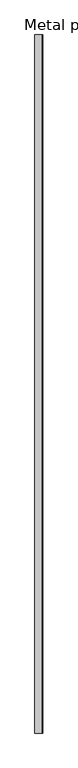
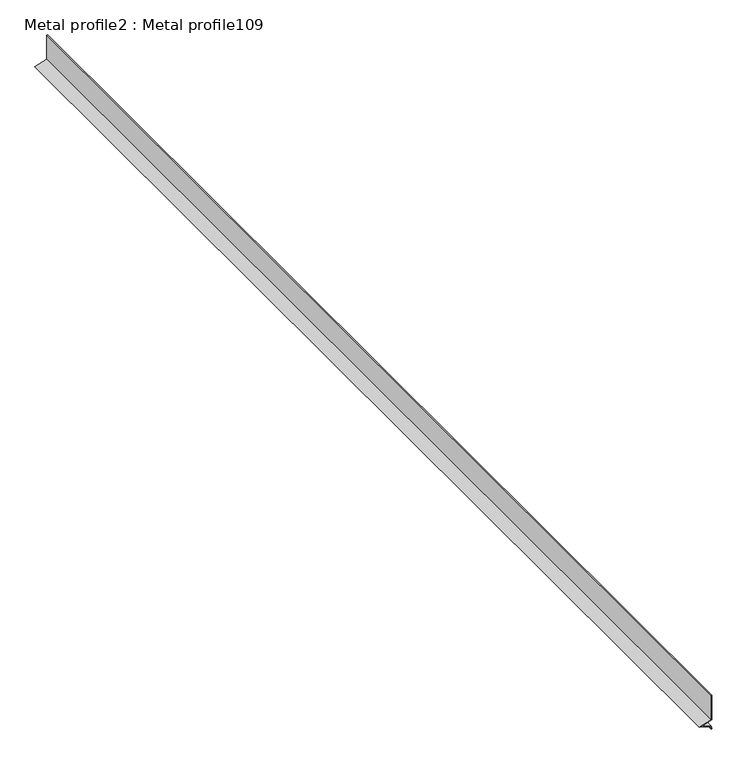
"""IFC4 building model written with IfcOpenShell, lengths in millimetres: proxy geometry, Metal profile2 : Metal profile109."""

from ifc_helpers import new_model, si_unit, frame, origin, place, context, project, spatial, polyline, outline, extrude, source, transform, mapped, element, save


def metal_profile2_metal_profile109_c648c6db(model_context):
    return source(origin(), model_context, "Body", "SweptSolid", [
        extrude(outline(polyline([(36749.8837679, 10041.7861998), (36754.9985183, 10040.8230047), (36760.4986763, 10023.7114021), (36766.3084327, 10041.7861998), (36811.2986763, 10041.7861998), (36811.2986763, 10040.5161998), (36767.234212, 10040.5161998), (36760.4986763, 10019.5611998), (36754.0207281, 10039.7148163), (36749.6487364, 10040.5381373), (36749.8837679, 10041.7861998)])), frame((0.0, 2217.3610563, 0.0), z_axis=(0.0, 1.0, 0.0), x_axis=(0.0, 0.0, 1.0)), (0.0, 0.0, 1.0), 2000.0),
    ])


if __name__ == "__main__":
    model = new_model("IFC4")
    model_context = context("Model", 3, world=origin())
    ifc_project = project(units=[si_unit("LENGTHUNIT", "METRE", prefix="MILLI")], contexts=[model_context])
    site = spatial("IfcSite", under=ifc_project)
    building = spatial("IfcBuilding", under=site)
    placement = place(None, origin())
    metal_profile2_metal_profile109_shape = metal_profile2_metal_profile109_c648c6db(model_context)
    element("IfcBuildingElementProxy", 1, Name="Metal profile2 : Metal profile109", ObjectType="Metal profile2 : Metal profile109", at=placement, inside=building, context=model_context, shape_type="MappedRepresentation", body=[
        mapped(metal_profile2_metal_profile109_shape, transform((0.0, 0.0, 0.0), x_axis=(1.0, 0.0, 0.0), y_axis=(0.0, 1.0, 0.0), z_axis=(0.0, 0.0, 1.0))),
    ])
    save(model, "model.ifc")

# Revit data of these elements
# Type "Metal profile2 : Metal profile109"
#   NameOverride = "Metal profile109"
# Element 1 (IfcBuildingElementProxy, "Metal profile2 : Metal profile109")
#   Materials on its faces: "16 GA. COPPER WEEP SCREED W/ MIN 3 1/2\" ATTACHMENT FLANGE - LAP UNDERLAYMENT OVER WEED SCREED"
# Materials
#   "16 GA. COPPER WEEP SCREED W/ MIN 3 1/2\" ATTACHMENT FLANGE - LAP UNDERLAYMENT OVER WEED SCREED": class "Unassigned", colour RGB 251 232 155, transparency 0, Cost = 0
